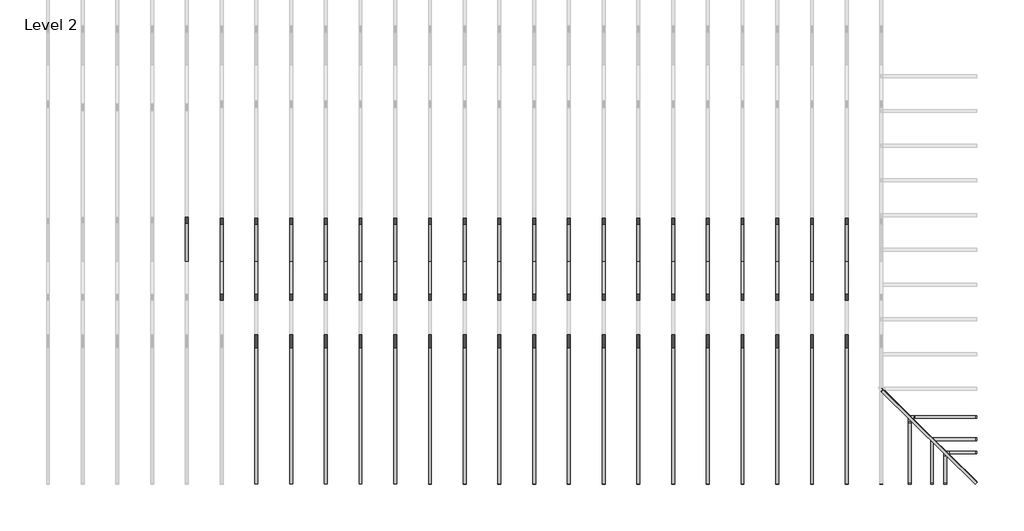
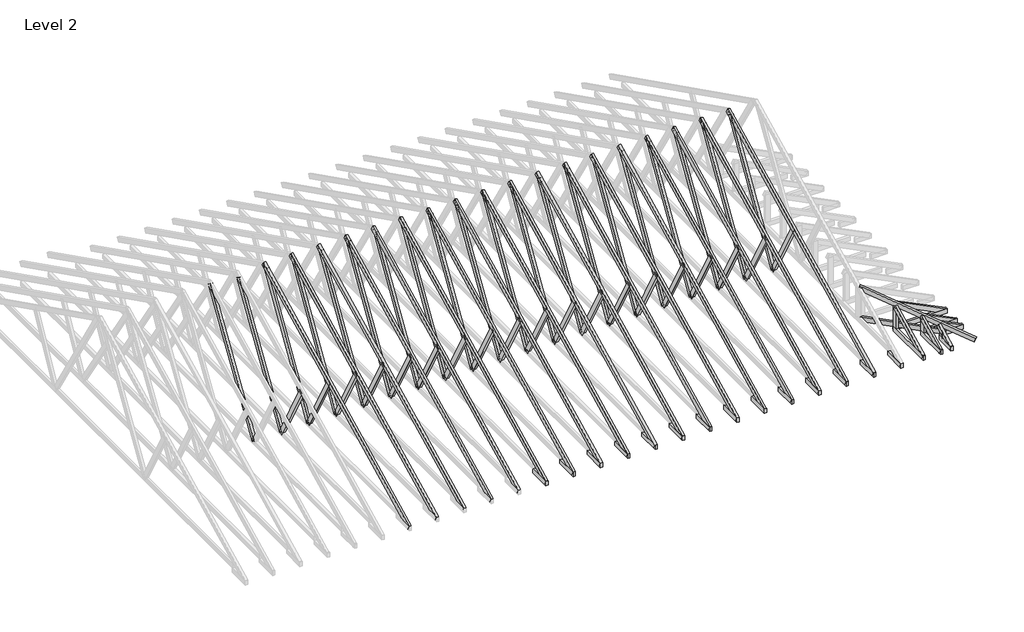
# One storey, part 2 of 5: 91 beams.
"""IFC4 building model written with IfcOpenShell, lengths in millimetres."""

import ifcopenshell
import ifcopenshell.guid

model = None  # the IFC model being written
_history = None  # IfcOwnerHistory: only IFC2X3 demands one
_inside = {}  # id of a spatial element -> (the spatial element, [elements in it])
_under = {}  # id of a project, library or spatial element -> (it, [spatial elements below it])
_declared = {}  # id of a project -> (the project, [libraries it declares])
_typed = {}  # id of a type object -> (the type object, [elements of that type])
_made_of = {}  # id of a material, layer set ... -> (it, [elements and type objects made of it])


def new_model(schema):
    """Start an empty IFC model of exactly this schema.

    Asked for "IFC4X3", IfcOpenShell would pick the latest addendum, in which some entities
    have other attributes; the version numbers below select the first issue.
    IFC2X3 requires an IfcOwnerHistory on every rooted entity: one is made here for all.
    """
    global model, _history
    if schema == "IFC4X3":
        model = ifcopenshell.file(schema_version=(4, 3, 0, 0))
    else:
        model = ifcopenshell.file(schema=schema)
    _inside.clear()
    _under.clear()
    _declared.clear()
    _typed.clear()
    _made_of.clear()
    _history = None
    if model.schema == "IFC2X3":
        org = make("IfcOrganization", Name="unknown")
        user = make(
            "IfcPersonAndOrganization",
            ThePerson=make("IfcPerson", FamilyName="unknown"),
            TheOrganization=org,
        )
        app = make(
            "IfcApplication",
            ApplicationDeveloper=org,
            Version="unknown",
            ApplicationFullName="unknown",
            ApplicationIdentifier="unknown",
        )
        _history = make(
            "IfcOwnerHistory",
            OwningUser=user,
            OwningApplication=app,
            ChangeAction="ADDED",
            CreationDate=0,
        )
    return model


def make(cls, **values):
    """One entity of the class cls with the attributes given. An attribute that is None is left unset."""
    return model.create_entity(
        cls, **{name: value for name, value in values.items() if value is not None}
    )


def rooted(cls, **values):
    """An entity with a GlobalId (a new one), such as an element, a storey or a relation."""
    return make(cls, GlobalId=ifcopenshell.guid.new(), OwnerHistory=_history, **values)


def si_unit(unit_type, name, prefix=None):
    """IfcSIUnit, for example si_unit("LENGTHUNIT", "METRE", prefix="MILLI")."""
    return make("IfcSIUnit", UnitType=unit_type, Prefix=prefix, Name=name)


def assignment(units):
    """IfcUnitAssignment: the units of a project."""
    return None if units is None else make("IfcUnitAssignment", Units=units)


def point(xyz):
    """IfcCartesianPoint."""
    return None if xyz is None else make("IfcCartesianPoint", Coordinates=xyz)


def direction(xyz):
    """IfcDirection."""
    return None if xyz is None else make("IfcDirection", DirectionRatios=xyz)


def frame(location, z_axis=None, x_axis=None):
    """IfcAxis2Placement3D, a coordinate frame: its origin and axes. An axis left out is left unset."""
    return make(
        "IfcAxis2Placement3D",
        Location=point(location),
        Axis=direction(z_axis),
        RefDirection=direction(x_axis),
    )


def origin():
    """The frame at (0, 0, 0) with its axes left unset."""
    return frame((0.0, 0.0, 0.0))


def place(relative_to, where):
    """IfcLocalPlacement: puts the frame where relative to a parent placement (None: the world)."""
    return make(
        "IfcLocalPlacement", PlacementRelTo=relative_to, RelativePlacement=where
    )


def context(
    kind, dimensions, precision=None, world=None, true_north=None, identifier=None
):
    """IfcGeometricRepresentationContext, for example the 3D "Model" context."""
    return make(
        "IfcGeometricRepresentationContext",
        ContextIdentifier=identifier,
        ContextType=kind,
        CoordinateSpaceDimension=dimensions,
        Precision=precision,
        WorldCoordinateSystem=world,
        TrueNorth=true_north,
    )


def project(units=None, contexts=None):
    """IfcProject with its units and contexts."""
    return rooted(
        "IfcProject",
        Name="project",
        RepresentationContexts=contexts,
        UnitsInContext=assignment(units),
    )


def spatial(cls, under=None, at=None, **own):
    """A site, building, storey or space (cls), placed at a placement, below another one or the project."""
    s = rooted(cls, ObjectPlacement=at, **own)
    if under is not None:
        _under.setdefault(under.id(), (under, []))[1].append(s)
    return s


def polyline(points):
    """IfcPolyline through the points."""
    return make("IfcPolyline", Points=[point(p) for p in points])


def outline(outer, holes=None, kind="AREA"):
    """IfcArbitraryClosedProfileDef: a profile drawn as a closed curve; with holes, ...WithVoids."""
    if holes is None:
        return make("IfcArbitraryClosedProfileDef", ProfileType=kind, OuterCurve=outer)
    return make(
        "IfcArbitraryProfileDefWithVoids",
        ProfileType=kind,
        OuterCurve=outer,
        InnerCurves=holes,
    )


def extrude(swept, where, along, depth):
    """IfcExtrudedAreaSolid: the profile swept, set in the frame where, extruded along a direction by depth."""
    return make(
        "IfcExtrudedAreaSolid",
        SweptArea=swept,
        Position=where,
        ExtrudedDirection=direction(along),
        Depth=depth,
    )


def shape(context_of_items, identifier, shape_type, items):
    """IfcShapeRepresentation: the items that make up one representation, for example the "Body"."""
    return make(
        "IfcShapeRepresentation",
        ContextOfItems=context_of_items,
        RepresentationIdentifier=identifier,
        RepresentationType=shape_type,
        Items=items,
    )


def source(mapping_origin, context_of_items, identifier, shape_type, items):
    """IfcRepresentationMap: a shape defined once, which mapped items show again and again."""
    return make(
        "IfcRepresentationMap",
        MappingOrigin=mapping_origin,
        MappedRepresentation=shape(context_of_items, identifier, shape_type, items),
    )


def transform(
    local_origin,
    x_axis=None,
    y_axis=None,
    z_axis=None,
    scale=None,
    scale2=None,
    scale3=None,
    uniform=True,
):
    """IfcCartesianTransformationOperator3D, or its non-uniform kind. x_axis, y_axis, z_axis: its Axis1, 2, 3."""
    if uniform:
        return make(
            "IfcCartesianTransformationOperator3D",
            Axis1=direction(x_axis),
            Axis2=direction(y_axis),
            LocalOrigin=point(local_origin),
            Scale=scale,
            Axis3=direction(z_axis),
        )
    return make(
        "IfcCartesianTransformationOperator3DnonUniform",
        Axis1=direction(x_axis),
        Axis2=direction(y_axis),
        LocalOrigin=point(local_origin),
        Scale=scale,
        Axis3=direction(z_axis),
        Scale2=scale2,
        Scale3=scale3,
    )


def mapped(mapping_source, mapping_target):
    """IfcMappedItem: shows the shape of a source again, moved by a transform."""
    return make(
        "IfcMappedItem", MappingSource=mapping_source, MappingTarget=mapping_target
    )


def made_of(thing, what):
    """Note that an element or type object is made of a material, layer set ...; save() writes the relation."""
    if what is not None:
        _made_of.setdefault(what.id(), (what, []))[1].append(thing)
    return thing


def element(
    cls,
    number,
    at=None,
    inside=None,
    cuts=None,
    type_object=None,
    material=None,
    context=None,
    identifier="Body",
    shape_type=None,
    held_by="IfcProductDefinitionShape",
    body=None,
    shapes=None,
    **own,
):
    """One element of the class cls, such as IfcWall. Its Tag is "e" and its number.

    at: its placement. inside: the storey or other place that contains it. cuts: it is an
    opening in that element (IfcRelVoidsElement). A single representation is given by context,
    identifier, shape_type and body (its items); several are given by shapes. held_by: the class
    of the entity that holds the representations. save() writes the other relations.
    """
    e = rooted(cls, Tag="e%d" % number, ObjectPlacement=at, **own)
    if body is not None:
        shapes = [shape(context, identifier, shape_type, body)]
    if shapes is not None:
        e.Representation = make(held_by, Representations=shapes)
    if inside is not None:
        _inside.setdefault(inside.id(), (inside, []))[1].append(e)
    if cuts is not None:
        rooted(
            "IfcRelVoidsElement", RelatingBuildingElement=cuts, RelatedOpeningElement=e
        )
    if type_object is not None:
        _typed.setdefault(type_object.id(), (type_object, []))[1].append(e)
    return made_of(e, material)


def aggregate(whole, parts):
    """IfcRelAggregates: a whole, such as a stair, and the parts it consists of."""
    return rooted("IfcRelAggregates", RelatingObject=whole, RelatedObjects=parts)


def save(model, path):
    """Write the relations noted so far, then the file.

    IfcRelAggregates (storeys below a building ...), IfcRelContainedInSpatialStructure (elements
    in a storey), IfcRelDefinesByType, IfcRelAssociatesMaterial and IfcRelDeclares: one each for
    every whole, place, type object, material and project.
    """
    for whole, parts in _under.values():
        aggregate(whole, parts)
    for where, things in _inside.values():
        rooted(
            "IfcRelContainedInSpatialStructure",
            RelatedElements=things,
            RelatingStructure=where,
        )
    for kind, things in _typed.values():
        rooted("IfcRelDefinesByType", RelatedObjects=things, RelatingType=kind)
    for what, things in _made_of.values():
        rooted("IfcRelAssociatesMaterial", RelatedObjects=things, RelatingMaterial=what)
    for by, libraries in _declared.values():
        rooted("IfcRelDeclares", RelatingContext=by, RelatedDefinitions=libraries)
    model.write(path)


def beam_3a1eac92(model_context):
    return source(origin(), model_context, "Body", "SweptSolid", [
        extrude(outline(polyline([(233.4866591, 25.4), (233.4866591, -25.4), (-1464.867127, -25.4), (-1464.867127, 25.4), (233.4866591, 25.4)])), frame((0.0, 0.0, -50.8), z_axis=(0.0, 0.0, 1.0), x_axis=(1.0, 0.0, 0.0)), (0.0, 0.0, 1.0), 101.6),
    ])


def beam_7745fe0f(model_context):
    return source(origin(), model_context, "Body", "SweptSolid", [
        extrude(outline(polyline([(393.7, 25.4), (393.7, -25.4), (-393.7, -25.4), (-393.7, 25.4), (393.7, 25.4)])), frame((0.0, 0.0, -50.8), z_axis=(0.0, 0.0, 1.0), x_axis=(1.0, 0.0, 0.0)), (0.0, 0.0, 1.0), 101.6),
    ])


def beam_54dd7b45(model_context):
    return source(origin(), model_context, "Body", "SweptSolid", [
        extrude(outline(polyline([(393.7, -25.4), (-368.3, -25.4), (-368.3, 25.4), (393.7, 25.4), (393.7, -25.4)])), frame((0.0, 0.0, -50.8), z_axis=(0.0, 0.0, 1.0), x_axis=(1.0, 0.0, 0.0)), (0.0, 0.0, 1.0), 101.6),
    ])


def beam_16181373(model_context):
    return source(origin(), model_context, "Body", "SweptSolid", [
        extrude(outline(polyline([(819.5010489, 25.4), (819.5010489, -25.4), (-821.193698, -25.4), (-821.193698, 25.4), (819.5010489, 25.4)])), frame((0.0, 0.0, -50.8), z_axis=(0.0, 0.0, 1.0), x_axis=(1.0, 0.0, 0.0)), (0.0, 0.0, 1.0), 101.6),
    ])


def beam_e838d316(model_context):
    return source(origin(), model_context, "Body", "SweptSolid", [
        extrude(outline(polyline([(1561.1045551, 25.4), (1561.1045551, -25.4), (-1572.5300502, -25.4), (-1572.5300502, 25.4), (1561.1045551, 25.4)])), frame((0.0, 0.0, -50.8), z_axis=(0.0, 0.0, 1.0), x_axis=(1.0, 0.0, 0.0)), (0.0, 0.0, 1.0), 101.6),
    ])


def beam_6a2c9f8f(model_context):
    return source(origin(), model_context, "Body", "SweptSolid", [
        extrude(outline(polyline([(1599.9543138, 25.4), (1599.9543138, -25.4), (-1584.2465686, -25.4), (-1584.2465686, 25.4), (1599.9543138, 25.4)])), frame((0.0, 0.0, -50.8), z_axis=(0.0, 0.0, 1.0), x_axis=(1.0, 0.0, 0.0)), (0.0, 0.0, 1.0), 101.6),
    ])


def beam_87710fdd(model_context):
    return source(origin(), model_context, "Body", "SweptSolid", [
        extrude(outline(polyline([(147.1272806, 25.4), (147.1272806, -25.4), (-142.875, -25.4), (-142.875, 25.4), (147.1272806, 25.4)])), frame((0.0, 0.0, -50.8), z_axis=(0.0, 0.0, 1.0), x_axis=(1.0, 0.0, 0.0)), (0.0, 0.0, 1.0), 101.6),
    ])


def beam_af5d22dc(model_context):
    return source(origin(), model_context, "Body", "SweptSolid", [
        extrude(outline(polyline([(571.5, 25.4), (571.5, -25.4), (-609.6, -25.4), (-609.6, 25.4), (571.5, 25.4)])), frame((0.0, 0.0, -50.8), z_axis=(0.0, 0.0, 1.0), x_axis=(1.0, 0.0, 0.0)), (0.0, 0.0, 1.0), 101.6),
    ])


def beam_7b8fa6d1(model_context):
    return source(origin(), model_context, "Body", "SweptSolid", [
        extrude(outline(polyline([(270.7395597, 25.4), (270.7395597, -25.4), (-219.9395597, -25.4), (-219.9395597, 25.4), (270.7395597, 25.4)])), frame((0.0, 0.0, -50.8), z_axis=(0.0, 0.0, 1.0), x_axis=(1.0, 0.0, 0.0)), (0.0, 0.0, 1.0), 101.6),
    ])


def beam_42a29ae5(model_context):
    return source(origin(), model_context, "Body", "SweptSolid", [
        extrude(outline(polyline([(270.7395597, -25.4), (-219.9395597, -25.4), (-219.9395597, 25.4), (270.7395597, 25.4), (270.7395597, -25.4)])), frame((0.0, 0.0, -50.8), z_axis=(0.0, 0.0, 1.0), x_axis=(1.0, 0.0, 0.0)), (0.0, 0.0, 1.0), 101.6),
    ])


def beam_11c5b8ca(model_context):
    return source(origin(), model_context, "Body", "SweptSolid", [
        extrude(outline(polyline([(147.1272806, -25.4), (-142.875, -25.4), (-142.875, 25.4), (147.1272806, 25.4), (147.1272806, -25.4)])), frame((0.0, 0.0, -50.8), z_axis=(0.0, 0.0, 1.0), x_axis=(1.0, 0.0, 0.0)), (0.0, 0.0, 1.0), 101.6),
    ])


def beam_5ac0b85f(model_context):
    return source(origin(), model_context, "Body", "SweptSolid", [
        extrude(outline(polyline([(571.5, -25.4), (-584.2, -25.4), (-584.2, 25.4), (571.5, 25.4), (571.5, -25.4)])), frame((0.0, 0.0, -50.8), z_axis=(0.0, 0.0, 1.0), x_axis=(1.0, 0.0, 0.0)), (0.0, 0.0, 1.0), 101.6),
    ])


def beam_ec111315(model_context):
    return source(origin(), model_context, "Body", "SweptSolid", [
        extrude(outline(polyline([(279.4, -25.4), (-228.6, -25.4), (-228.6, 25.4), (279.4, 25.4), (279.4, -25.4)])), frame((0.0, 0.0, -50.8), z_axis=(0.0, 0.0, 1.0), x_axis=(1.0, 0.0, 0.0)), (0.0, 0.0, 1.0), 101.6),
    ])


def beam_878446a4(model_context):
    return source(origin(), model_context, "Body", "SweptSolid", [
        extrude(outline(polyline([(63.8057136, 25.4), (63.8057136, -25.4), (-59.553433, -25.4), (-59.553433, 25.4), (63.8057136, 25.4)])), frame((0.0, 0.0, -50.8), z_axis=(0.0, 0.0, 1.0), x_axis=(1.0, 0.0, 0.0)), (0.0, 0.0, 1.0), 101.6),
    ])


def beam_bc99fd75(model_context):
    return source(origin(), model_context, "Body", "SweptSolid", [
        extrude(outline(polyline([(222.3387319, 25.4), (222.3387319, -25.4), (-231.775, -25.4), (-231.775, 25.4), (222.3387319, 25.4)])), frame((0.0, 0.0, -50.8), z_axis=(0.0, 0.0, 1.0), x_axis=(1.0, 0.0, 0.0)), (0.0, 0.0, 1.0), 101.6),
    ])


def beam_efe25585(model_context):
    return source(origin(), model_context, "Body", "SweptSolid", [
        extrude(outline(polyline([(222.3387319, -25.4), (-231.775, -25.4), (-231.775, 25.4), (222.3387319, 25.4), (222.3387319, -25.4)])), frame((0.0, 0.0, -50.8), z_axis=(0.0, 0.0, 1.0), x_axis=(1.0, 0.0, 0.0)), (0.0, 0.0, 1.0), 101.6),
    ])


def beam_dfed05dc(model_context):
    return source(origin(), model_context, "Body", "SweptSolid", [
        extrude(outline(polyline([(63.8057136, -25.4), (-59.553433, -25.4), (-59.553433, 25.4), (63.8057136, 25.4), (63.8057136, -25.4)])), frame((0.0, 0.0, -50.8), z_axis=(0.0, 0.0, 1.0), x_axis=(1.0, 0.0, 0.0)), (0.0, 0.0, 1.0), 101.6),
    ])


model = new_model("IFC4")

# Units and contexts
model_context = context("Model", 3, world=origin())
ifc_project = project(units=[si_unit("LENGTHUNIT", "METRE", prefix="MILLI")], contexts=[model_context])

# Site, building, storey
site = spatial("IfcSite", under=ifc_project)
building = spatial("IfcBuilding", under=site)
storey = spatial("IfcBuildingStorey", under=building, Name="Level 2", Elevation=2768.6)

# Beams
placement = place(None, origin())
element("IfcBeam", 1, ObjectType="Dimension Lumber : BLDG 6241 2X4\" TRUSS MEMBER", at=placement, inside=storey, context=model_context, shape_type="SweptSolid", body=[
    extrude(outline(polyline([(0.0, -50.8), (0.0, 0.0), (6302.3539791, 0.0), (6302.3539791, -50.8), (0.0, -50.8)])), frame((-10511.414829, -5565.5155384, 2678.5857718), z_axis=(0.0, -0.447213595499958, 0.894427190999916), x_axis=(0.0, 0.894427190999916, 0.447213595499958)), (0.0, 0.0, 1.0), 101.6),
])
element("IfcBeam", 2, ObjectType="Dimension Lumber : BLDG 6241 2X4\" TRUSS MEMBER", at=placement, inside=storey, context=model_context, shape_type="SweptSolid", body=[
    extrude(outline(polyline([(0.0, -50.8), (0.0, 0.0), (6302.3539791, 0.0), (6302.3539791, -50.8), (0.0, -50.8)])), frame((-9901.814829, -5565.5155384, 2678.5857718), z_axis=(0.0, -0.447213595499958, 0.894427190999916), x_axis=(0.0, 0.894427190999916, 0.447213595499958)), (0.0, 0.0, 1.0), 101.6),
])
element("IfcBeam", 3, ObjectType="Dimension Lumber : BLDG 6241 2X4\" TRUSS MEMBER", at=placement, inside=storey, context=model_context, shape_type="SweptSolid", body=[
    extrude(outline(polyline([(0.0, -50.8), (0.0, 0.0), (6302.3539791, 0.0), (6302.3539791, -50.8), (0.0, -50.8)])), frame((-9292.214829, -5565.5155384, 2678.5857718), z_axis=(0.0, -0.447213595499958, 0.894427190999916), x_axis=(0.0, 0.894427190999916, 0.447213595499958)), (0.0, 0.0, 1.0), 101.6),
])
element("IfcBeam", 4, ObjectType="Dimension Lumber : BLDG 6241 2X4\" TRUSS MEMBER", at=placement, inside=storey, context=model_context, shape_type="SweptSolid", body=[
    extrude(outline(polyline([(0.0, -50.8), (0.0, 0.0), (6302.3539791, 0.0), (6302.3539791, -50.8), (0.0, -50.8)])), frame((-8682.614829, -5565.5155384, 2678.5857718), z_axis=(0.0, -0.447213595499958, 0.894427190999916), x_axis=(0.0, 0.894427190999916, 0.447213595499958)), (0.0, 0.0, 1.0), 101.6),
])
element("IfcBeam", 5, ObjectType="Dimension Lumber : BLDG 6241 2X4\" TRUSS MEMBER", at=placement, inside=storey, context=model_context, shape_type="SweptSolid", body=[
    extrude(outline(polyline([(0.0, -50.8), (0.0, 0.0), (6302.3539791, 0.0), (6302.3539791, -50.8), (0.0, -50.8)])), frame((-8073.014829, -5565.5155384, 2678.5857718), z_axis=(0.0, -0.447213595499958, 0.894427190999916), x_axis=(0.0, 0.894427190999916, 0.447213595499958)), (0.0, 0.0, 1.0), 101.6),
])
element("IfcBeam", 6, ObjectType="Dimension Lumber : BLDG 6241 2X4\" TRUSS MEMBER", at=placement, inside=storey, context=model_context, shape_type="SweptSolid", body=[
    extrude(outline(polyline([(0.0, -50.8), (0.0, 0.0), (6302.3539791, 0.0), (6302.3539791, -50.8), (0.0, -50.8)])), frame((-7463.414829, -5565.5155384, 2678.5857718), z_axis=(0.0, -0.447213595499958, 0.8944271909999159), x_axis=(0.0, 0.8944271909999159, 0.447213595499958)), (0.0, 0.0, 1.0), 101.6),
])
element("IfcBeam", 7, ObjectType="Dimension Lumber : BLDG 6241 2X4\" TRUSS MEMBER", at=placement, inside=storey, context=model_context, shape_type="SweptSolid", body=[
    extrude(outline(polyline([(0.0, -50.8), (0.0, 0.0), (6302.3539791, 0.0), (6302.3539791, -50.8), (0.0, -50.8)])), frame((-6853.814829, -5565.5155384, 2678.5857718), z_axis=(0.0, -0.44721359549995776, 0.894427190999916), x_axis=(0.0, 0.894427190999916, 0.44721359549995776)), (0.0, 0.0, 1.0), 101.6),
])
element("IfcBeam", 8, ObjectType="Dimension Lumber : BLDG 6241 2X4\" TRUSS MEMBER", at=placement, inside=storey, context=model_context, shape_type="SweptSolid", body=[
    extrude(outline(polyline([(0.0, -50.8), (0.0, 0.0), (6302.3539791, 0.0), (6302.3539791, -50.8), (0.0, -50.8)])), frame((-6244.214829, -5565.5155384, 2678.5857718), z_axis=(0.0, -0.447213595499958, 0.894427190999916), x_axis=(0.0, 0.894427190999916, 0.447213595499958)), (0.0, 0.0, 1.0), 101.6),
])
element("IfcBeam", 9, ObjectType="Dimension Lumber : BLDG 6241 2X4\" TRUSS MEMBER", at=placement, inside=storey, context=model_context, shape_type="SweptSolid", body=[
    extrude(outline(polyline([(0.0, -50.8), (0.0, 0.0), (6302.3539791, 0.0), (6302.3539791, -50.8), (0.0, -50.8)])), frame((-5634.614829, -5565.5155384, 2678.5857718), z_axis=(0.0, -0.447213595499958, 0.894427190999916), x_axis=(0.0, 0.894427190999916, 0.447213595499958)), (0.0, 0.0, 1.0), 101.6),
])
element("IfcBeam", 10, ObjectType="Dimension Lumber : BLDG 6241 2X4\" TRUSS MEMBER", at=placement, inside=storey, context=model_context, shape_type="SweptSolid", body=[
    extrude(outline(polyline([(0.0, -50.8), (0.0, 0.0), (6302.3539791, 0.0), (6302.3539791, -50.8), (0.0, -50.8)])), frame((-5025.014829, -5565.5155384, 2678.5857718), z_axis=(0.0, -0.447213595499958, 0.894427190999916), x_axis=(0.0, 0.894427190999916, 0.447213595499958)), (0.0, 0.0, 1.0), 101.6),
])
element("IfcBeam", 11, ObjectType="Dimension Lumber : BLDG 6241 2X4\" TRUSS MEMBER", at=placement, inside=storey, context=model_context, shape_type="SweptSolid", body=[
    extrude(outline(polyline([(0.0, -50.8), (0.0, 0.0), (6302.3539791, 0.0), (6302.3539791, -50.8), (0.0, -50.8)])), frame((-4415.414829, -5565.5155384, 2678.5857718), z_axis=(0.0, -0.447213595499958, 0.894427190999916), x_axis=(0.0, 0.894427190999916, 0.447213595499958)), (0.0, 0.0, 1.0), 101.6),
])
element("IfcBeam", 12, ObjectType="Dimension Lumber : BLDG 6241 2X4\" TRUSS MEMBER", at=placement, inside=storey, context=model_context, shape_type="SweptSolid", body=[
    extrude(outline(polyline([(0.0, -50.8), (0.0, 0.0), (6302.3539791, 0.0), (6302.3539791, -50.8), (0.0, -50.8)])), frame((-3805.814829, -5565.5155384, 2678.5857718), z_axis=(0.0, -0.447213595499958, 0.894427190999916), x_axis=(0.0, 0.894427190999916, 0.447213595499958)), (0.0, 0.0, 1.0), 101.6),
])
element("IfcBeam", 13, ObjectType="Dimension Lumber : BLDG 6241 2X4\" TRUSS MEMBER", at=placement, inside=storey, context=model_context, shape_type="SweptSolid", body=[
    extrude(outline(polyline([(0.0, -50.8), (0.0, 0.0), (6302.3539791, 0.0), (6302.3539791, -50.8), (0.0, -50.8)])), frame((-3196.214829, -5565.5155384, 2678.5857718), z_axis=(0.0, -0.447213595499958, 0.894427190999916), x_axis=(0.0, 0.894427190999916, 0.447213595499958)), (0.0, 0.0, 1.0), 101.6),
])
element("IfcBeam", 14, ObjectType="Dimension Lumber : BLDG 6241 2X4\" TRUSS MEMBER", at=placement, inside=storey, context=model_context, shape_type="SweptSolid", body=[
    extrude(outline(polyline([(0.0, -50.8), (0.0, 0.0), (6302.3539791, 0.0), (6302.3539791, -50.8), (0.0, -50.8)])), frame((-2586.614829, -5565.5155384, 2678.5857718), z_axis=(0.0, -0.447213595499958, 0.894427190999916), x_axis=(0.0, 0.894427190999916, 0.447213595499958)), (0.0, 0.0, 1.0), 101.6),
])
element("IfcBeam", 15, ObjectType="Dimension Lumber : BLDG 6241 2X4\" TRUSS MEMBER", at=placement, inside=storey, context=model_context, shape_type="SweptSolid", body=[
    extrude(outline(polyline([(0.0, -50.8), (0.0, 0.0), (6302.3539791, 0.0), (6302.3539791, -50.8), (0.0, -50.8)])), frame((-1977.014829, -5565.5155384, 2678.5857718), z_axis=(0.0, -0.447213595499958, 0.894427190999916), x_axis=(0.0, 0.894427190999916, 0.447213595499958)), (0.0, 0.0, 1.0), 101.6),
])
element("IfcBeam", 16, ObjectType="Dimension Lumber : BLDG 6241 2X4\" TRUSS MEMBER", at=placement, inside=storey, context=model_context, shape_type="SweptSolid", body=[
    extrude(outline(polyline([(0.0, -50.8), (0.0, 0.0), (6302.3539791, 0.0), (6302.3539791, -50.8), (0.0, -50.8)])), frame((-1367.414829, -5565.5155384, 2678.5857718), z_axis=(0.0, -0.447213595499958, 0.894427190999916), x_axis=(0.0, 0.894427190999916, 0.447213595499958)), (0.0, 0.0, 1.0), 101.6),
])
element("IfcBeam", 17, ObjectType="Dimension Lumber : BLDG 6241 2X4\" TRUSS MEMBER", at=placement, inside=storey, context=model_context, shape_type="SweptSolid", body=[
    extrude(outline(polyline([(0.0, -50.8), (0.0, 0.0), (6302.3539791, 0.0), (6302.3539791, -50.8), (0.0, -50.8)])), frame((-757.814829, -5565.5155384, 2678.5857718), z_axis=(0.0, -0.447213595499958, 0.8944271909999159), x_axis=(0.0, 0.8944271909999159, 0.447213595499958)), (0.0, 0.0, 1.0), 101.6),
])
element("IfcBeam", 18, ObjectType="Dimension Lumber : BLDG 6241 2X4\" TRUSS MEMBER", at=placement, inside=storey, context=model_context, shape_type="SweptSolid", body=[
    extrude(outline(polyline([(0.0, -50.8), (0.0, 0.0), (6302.3539791, 0.0), (6302.3539791, -50.8), (0.0, -50.8)])), frame((-148.214829, -5565.5155384, 2678.5857718), z_axis=(0.0, -0.44721359549995776, 0.894427190999916), x_axis=(0.0, 0.894427190999916, 0.44721359549995776)), (0.0, 0.0, 1.0), 101.6),
])
element("IfcBeam", 19, ObjectType="Dimension Lumber : BLDG 6241 2X4\" TRUSS MEMBER", at=placement, inside=storey, context=model_context, shape_type="SweptSolid", body=[
    extrude(outline(polyline([(0.0, -50.8000001), (0.0, 0.0), (2461.5286969, -1e-07), (2461.5286969, -50.8), (0.0, -50.8000001)])), frame((497.0810747, -3923.9012552, 3516.9362486), z_axis=(0.22183093198504453, -0.25320527715849106, 0.9416358772018718), x_axis=(0.6716162760239294, -0.6604274920267077, -0.3358081380119639)), (0.0, 0.0, 1.0), 101.6),
])
element("IfcBeam", 20, ObjectType="Dimension Lumber : BLDG 6241 2X4\" TRUSS MEMBER", at=placement, inside=storey, context=model_context, shape_type="SweptSolid", body=[
    extrude(outline(polyline([(0.0, -50.8), (0.0, 0.0), (1203.6219076, 0.0), (1203.6219076, -50.8), (0.0, -50.8)])), frame((2112.5153243, -4456.9715886, 2680.3426701), z_axis=(0.44721359549995937, 0.0, 0.8944271909999152), x_axis=(-0.8944271909999152, 0.0, 0.44721359549995937)), (0.0, 0.0, 1.0), 101.6),
])
element("IfcBeam", 21, ObjectType="Dimension Lumber : BLDG 6241 2X4\" TRUSS MEMBER", at=placement, inside=storey, context=model_context, shape_type="SweptSolid", body=[
    extrude(outline(polyline([(0.0, -50.8), (0.0, 0.0), (844.55, 0.0), (844.55, -50.8), (0.0, -50.8)])), frame((2117.2589031, -4850.6715886, 2677.9708807), z_axis=(0.4472135954999599, 0.0, 0.894427190999915), x_axis=(-0.894427190999915, 0.0, 0.4472135954999599)), (0.0, 0.0, 1.0), 101.6),
])
element("IfcBeam", 22, ObjectType="Dimension Lumber : BLDG 6241 2X4\" TRUSS MEMBER", at=placement, inside=storey, context=model_context, shape_type="SweptSolid", body=[
    extrude(outline(polyline([(0.0, 50.8), (1203.6219076, 50.8), (1203.6219076, 0.0), (0.0, 0.0), (0.0, 50.8)])), frame((1007.485171, -5562.001742, 2680.3426701), z_axis=(0.0, -0.44721359549995937, 0.8944271909999152), x_axis=(0.0, 0.8944271909999152, 0.44721359549995937)), (0.0, 0.0, 1.0), 101.6),
])
element("IfcBeam", 23, ObjectType="Dimension Lumber : BLDG 6241 2X4\" TRUSS MEMBER", at=placement, inside=storey, context=model_context, shape_type="SweptSolid", body=[
    extrude(outline(polyline([(0.0, 50.8), (844.55, 50.8), (844.55, 0.0), (0.0, 0.0), (0.0, 50.8)])), frame((1401.185171, -5566.7453207, 2677.9708807), z_axis=(0.0, -0.4472135954999599, 0.894427190999915), x_axis=(0.0, 0.894427190999915, 0.4472135954999599)), (0.0, 0.0, 1.0), 101.6),
])
element("IfcBeam", 24, ObjectType="Dimension Lumber : BLDG 6241 2X4\" TRUSS MEMBER", at=placement, inside=storey, context=model_context, shape_type="SweptSolid", body=[
    extrude(outline(polyline([(0.0, -50.8), (0.0, 0.0), (546.1, 0.0), (546.1, -50.8), (0.0, -50.8)])), frame((2116.9461224, -5079.2715886, 2678.127271), z_axis=(0.4472135954999593, 0.0, 0.8944271909999153), x_axis=(-0.8944271909999153, 0.0, 0.4472135954999593)), (0.0, 0.0, 1.0), 101.6),
])
element("IfcBeam", 25, ObjectType="Dimension Lumber : BLDG 6241 2X4\" TRUSS MEMBER", at=placement, inside=storey, context=model_context, shape_type="SweptSolid", body=[
    extrude(outline(polyline([(0.0, 50.8), (546.1, 50.8), (546.1, 0.0), (0.0, 0.0), (0.0, 50.8)])), frame((1629.785171, -5566.43254, 2678.127271), z_axis=(0.0, -0.4472135954999592, 0.8944271909999153), x_axis=(0.0, 0.8944271909999153, 0.4472135954999592)), (0.0, 0.0, 1.0), 101.6),
])
beam_shape = beam_3a1eac92(model_context)
element("IfcBeam", 26, ObjectType="Dimension Lumber : BLDG 6241 2X4\" TRUSS MEMBER", at=placement, inside=storey, context=model_context, shape_type="MappedRepresentation", body=[
    mapped(beam_shape, transform((677.285171, -4126.7715886, 2819.4), x_axis=(-0.7071067811865508, 0.7071067811865442, 0.0), y_axis=(-0.7071067811865442, -0.7071067811865508, 0.0), z_axis=(0.0, 0.0, 1.0))),
])
beam_2_shape = beam_7745fe0f(model_context)
element("IfcBeam", 27, ObjectType="Dimension Lumber : BLDG 6241 2X4\" TRUSS MEMBER", at=placement, inside=storey, context=model_context, shape_type="MappedRepresentation", body=[
    mapped(beam_2_shape, transform((1769.485171, -4825.2715886, 2728.7708807), x_axis=(1.0, 0.0, 0.0), y_axis=(0.0, 1.0, 0.0), z_axis=(0.0, 0.0, 1.0))),
])
beam_3_shape = beam_54dd7b45(model_context)
element("IfcBeam", 28, ObjectType="Dimension Lumber : BLDG 6241 2X4\" TRUSS MEMBER", at=placement, inside=storey, context=model_context, shape_type="MappedRepresentation", body=[
    mapped(beam_3_shape, transform((1375.785171, -5218.9715886, 2728.7708807), x_axis=(0.0, -1.0, 0.0), y_axis=(1.0, 0.0, 0.0), z_axis=(0.0, 0.0, 1.0))),
])
beam_4_shape = beam_16181373(model_context)
element("IfcBeam", 29, ObjectType="Dimension Lumber : BLDG 6241 2X4\" TRUSS MEMBER", at=placement, inside=storey, context=model_context, shape_type="MappedRepresentation", body=[
    mapped(beam_4_shape, transform((-11095.614829, -2095.6213634, 3552.5770493), x_axis=(0.0, -0.4803172630852174, 0.8770948220017754), y_axis=(-1.0, 0.0, 0.0), z_axis=(0.0, -0.8770948220017754, -0.4803172630852174))),
])
element("IfcBeam", 30, ObjectType="Dimension Lumber : BLDG 6241 2X4\" TRUSS MEMBER", at=placement, inside=storey, context=model_context, shape_type="MappedRepresentation", body=[
    mapped(beam_4_shape, transform((-10486.014829, -2095.6213634, 3552.5770493), x_axis=(0.0, -0.4803172630852174, 0.8770948220017754), y_axis=(-1.0, 0.0, 0.0), z_axis=(0.0, -0.8770948220017754, -0.4803172630852174))),
])
element("IfcBeam", 31, ObjectType="Dimension Lumber : BLDG 6241 2X4\" TRUSS MEMBER", at=placement, inside=storey, context=model_context, shape_type="MappedRepresentation", body=[
    mapped(beam_4_shape, transform((-9876.414829, -2095.6213634, 3552.5770493), x_axis=(0.0, -0.4803172630852174, 0.8770948220017754), y_axis=(-1.0, 0.0, 0.0), z_axis=(0.0, -0.8770948220017754, -0.4803172630852174))),
])
element("IfcBeam", 32, ObjectType="Dimension Lumber : BLDG 6241 2X4\" TRUSS MEMBER", at=placement, inside=storey, context=model_context, shape_type="MappedRepresentation", body=[
    mapped(beam_4_shape, transform((-9266.814829, -2095.6213634, 3552.5770493), x_axis=(0.0, -0.4803172630852174, 0.8770948220017754), y_axis=(-1.0, 0.0, 0.0), z_axis=(0.0, -0.8770948220017754, -0.4803172630852174))),
])
element("IfcBeam", 33, ObjectType="Dimension Lumber : BLDG 6241 2X4\" TRUSS MEMBER", at=placement, inside=storey, context=model_context, shape_type="MappedRepresentation", body=[
    mapped(beam_4_shape, transform((-8657.214829, -2095.6213634, 3552.5770493), x_axis=(0.0, -0.4803172630852174, 0.8770948220017754), y_axis=(-1.0, 0.0, 0.0), z_axis=(0.0, -0.8770948220017754, -0.4803172630852174))),
])
element("IfcBeam", 34, ObjectType="Dimension Lumber : BLDG 6241 2X4\" TRUSS MEMBER", at=placement, inside=storey, context=model_context, shape_type="MappedRepresentation", body=[
    mapped(beam_4_shape, transform((-8047.614829, -2095.6213634, 3552.5770493), x_axis=(0.0, -0.4803172630852174, 0.8770948220017754), y_axis=(-1.0, 0.0, 0.0), z_axis=(0.0, -0.8770948220017754, -0.4803172630852174))),
])
element("IfcBeam", 35, ObjectType="Dimension Lumber : BLDG 6241 2X4\" TRUSS MEMBER", at=placement, inside=storey, context=model_context, shape_type="MappedRepresentation", body=[
    mapped(beam_4_shape, transform((-7438.014829, -2095.6213634, 3552.5770493), x_axis=(0.0, -0.4803172630852174, 0.8770948220017754), y_axis=(-1.0, 0.0, 0.0), z_axis=(0.0, -0.8770948220017754, -0.4803172630852174))),
])
element("IfcBeam", 36, ObjectType="Dimension Lumber : BLDG 6241 2X4\" TRUSS MEMBER", at=placement, inside=storey, context=model_context, shape_type="MappedRepresentation", body=[
    mapped(beam_4_shape, transform((-6828.414829, -2095.6213634, 3552.5770493), x_axis=(0.0, -0.4803172630852174, 0.8770948220017754), y_axis=(-1.0, 0.0, 0.0), z_axis=(0.0, -0.8770948220017754, -0.4803172630852174))),
])
element("IfcBeam", 37, ObjectType="Dimension Lumber : BLDG 6241 2X4\" TRUSS MEMBER", at=placement, inside=storey, context=model_context, shape_type="MappedRepresentation", body=[
    mapped(beam_4_shape, transform((-6218.814829, -2095.6213634, 3552.5770493), x_axis=(0.0, -0.4803172630852174, 0.8770948220017754), y_axis=(-1.0, 0.0, 0.0), z_axis=(0.0, -0.8770948220017754, -0.4803172630852174))),
])
element("IfcBeam", 38, ObjectType="Dimension Lumber : BLDG 6241 2X4\" TRUSS MEMBER", at=placement, inside=storey, context=model_context, shape_type="MappedRepresentation", body=[
    mapped(beam_4_shape, transform((-5609.214829, -2095.6213634, 3552.5770493), x_axis=(0.0, -0.4803172630852174, 0.8770948220017754), y_axis=(-1.0, 0.0, 0.0), z_axis=(0.0, -0.8770948220017754, -0.4803172630852174))),
])
element("IfcBeam", 39, ObjectType="Dimension Lumber : BLDG 6241 2X4\" TRUSS MEMBER", at=placement, inside=storey, context=model_context, shape_type="MappedRepresentation", body=[
    mapped(beam_4_shape, transform((-4999.614829, -2095.6213634, 3552.5770493), x_axis=(0.0, -0.4803172630852174, 0.8770948220017754), y_axis=(-1.0, 0.0, 0.0), z_axis=(0.0, -0.8770948220017754, -0.4803172630852174))),
])
element("IfcBeam", 40, ObjectType="Dimension Lumber : BLDG 6241 2X4\" TRUSS MEMBER", at=placement, inside=storey, context=model_context, shape_type="MappedRepresentation", body=[
    mapped(beam_4_shape, transform((-4390.014829, -2095.6213634, 3552.5770493), x_axis=(0.0, -0.4803172630852174, 0.8770948220017754), y_axis=(-1.0, 0.0, 0.0), z_axis=(0.0, -0.8770948220017754, -0.4803172630852174))),
])
element("IfcBeam", 41, ObjectType="Dimension Lumber : BLDG 6241 2X4\" TRUSS MEMBER", at=placement, inside=storey, context=model_context, shape_type="MappedRepresentation", body=[
    mapped(beam_4_shape, transform((-3780.414829, -2095.6213634, 3552.5770493), x_axis=(0.0, -0.4803172630852174, 0.8770948220017754), y_axis=(-1.0, 0.0, 0.0), z_axis=(0.0, -0.8770948220017754, -0.4803172630852174))),
])
element("IfcBeam", 42, ObjectType="Dimension Lumber : BLDG 6241 2X4\" TRUSS MEMBER", at=placement, inside=storey, context=model_context, shape_type="MappedRepresentation", body=[
    mapped(beam_4_shape, transform((-3170.814829, -2095.6213634, 3552.5770493), x_axis=(0.0, -0.4803172630852174, 0.8770948220017754), y_axis=(-1.0, 0.0, 0.0), z_axis=(0.0, -0.8770948220017754, -0.4803172630852174))),
])
element("IfcBeam", 43, ObjectType="Dimension Lumber : BLDG 6241 2X4\" TRUSS MEMBER", at=placement, inside=storey, context=model_context, shape_type="MappedRepresentation", body=[
    mapped(beam_4_shape, transform((-2561.214829, -2095.6213634, 3552.5770493), x_axis=(0.0, -0.4803172630852174, 0.8770948220017754), y_axis=(-1.0, 0.0, 0.0), z_axis=(0.0, -0.8770948220017754, -0.4803172630852174))),
])
element("IfcBeam", 44, ObjectType="Dimension Lumber : BLDG 6241 2X4\" TRUSS MEMBER", at=placement, inside=storey, context=model_context, shape_type="MappedRepresentation", body=[
    mapped(beam_4_shape, transform((-1951.614829, -2095.6213634, 3552.5770493), x_axis=(0.0, -0.4803172630852174, 0.8770948220017754), y_axis=(-1.0, 0.0, 0.0), z_axis=(0.0, -0.8770948220017754, -0.4803172630852174))),
])
element("IfcBeam", 45, ObjectType="Dimension Lumber : BLDG 6241 2X4\" TRUSS MEMBER", at=placement, inside=storey, context=model_context, shape_type="MappedRepresentation", body=[
    mapped(beam_4_shape, transform((-1342.014829, -2095.6213634, 3552.5770493), x_axis=(0.0, -0.4803172630852174, 0.8770948220017754), y_axis=(-1.0, 0.0, 0.0), z_axis=(0.0, -0.8770948220017754, -0.4803172630852174))),
])
element("IfcBeam", 46, ObjectType="Dimension Lumber : BLDG 6241 2X4\" TRUSS MEMBER", at=placement, inside=storey, context=model_context, shape_type="MappedRepresentation", body=[
    mapped(beam_4_shape, transform((-732.414829, -2095.6213634, 3552.5770493), x_axis=(0.0, -0.4803172630852174, 0.8770948220017754), y_axis=(-1.0, 0.0, 0.0), z_axis=(0.0, -0.8770948220017754, -0.4803172630852174))),
])
element("IfcBeam", 47, ObjectType="Dimension Lumber : BLDG 6241 2X4\" TRUSS MEMBER", at=placement, inside=storey, context=model_context, shape_type="MappedRepresentation", body=[
    mapped(beam_4_shape, transform((-122.814829, -2095.6213634, 3552.5770493), x_axis=(0.0, -0.4803172630852174, 0.8770948220017754), y_axis=(-1.0, 0.0, 0.0), z_axis=(0.0, -0.8770948220017754, -0.4803172630852174))),
])
beam_5_shape = beam_e838d316(model_context)
element("IfcBeam", 48, ObjectType="Dimension Lumber : BLDG 6241 2X4\" TRUSS MEMBER", at=placement, inside=storey, context=model_context, shape_type="MappedRepresentation", body=[
    mapped(beam_5_shape, transform((-11095.614829, -880.0831247, 4160.3461686), x_axis=(0.0, -0.5257715142502325, -0.8506258371358218), y_axis=(-1.0, 0.0, 0.0), z_axis=(0.0, 0.8506258371358218, -0.5257715142502325))),
])
element("IfcBeam", 49, ObjectType="Dimension Lumber : BLDG 6241 2X4\" TRUSS MEMBER", at=placement, inside=storey, context=model_context, shape_type="MappedRepresentation", body=[
    mapped(beam_5_shape, transform((-10486.014829, -880.0831247, 4160.3461686), x_axis=(0.0, -0.5257715142502325, -0.8506258371358218), y_axis=(-1.0, 0.0, 0.0), z_axis=(0.0, 0.8506258371358218, -0.5257715142502325))),
])
element("IfcBeam", 50, ObjectType="Dimension Lumber : BLDG 6241 2X4\" TRUSS MEMBER", at=placement, inside=storey, context=model_context, shape_type="MappedRepresentation", body=[
    mapped(beam_5_shape, transform((-9876.414829, -880.0831247, 4160.3461686), x_axis=(0.0, -0.5257715142502325, -0.8506258371358218), y_axis=(-1.0, 0.0, 0.0), z_axis=(0.0, 0.8506258371358218, -0.5257715142502325))),
])
element("IfcBeam", 51, ObjectType="Dimension Lumber : BLDG 6241 2X4\" TRUSS MEMBER", at=placement, inside=storey, context=model_context, shape_type="MappedRepresentation", body=[
    mapped(beam_5_shape, transform((-9266.814829, -880.0831247, 4160.3461686), x_axis=(0.0, -0.5257715142502325, -0.8506258371358218), y_axis=(-1.0, 0.0, 0.0), z_axis=(0.0, 0.8506258371358218, -0.5257715142502325))),
])
element("IfcBeam", 52, ObjectType="Dimension Lumber : BLDG 6241 2X4\" TRUSS MEMBER", at=placement, inside=storey, context=model_context, shape_type="MappedRepresentation", body=[
    mapped(beam_5_shape, transform((-8657.214829, -880.0831247, 4160.3461686), x_axis=(0.0, -0.5257715142502325, -0.8506258371358218), y_axis=(-1.0, 0.0, 0.0), z_axis=(0.0, 0.8506258371358218, -0.5257715142502325))),
])
element("IfcBeam", 53, ObjectType="Dimension Lumber : BLDG 6241 2X4\" TRUSS MEMBER", at=placement, inside=storey, context=model_context, shape_type="MappedRepresentation", body=[
    mapped(beam_5_shape, transform((-8047.614829, -880.0831247, 4160.3461686), x_axis=(0.0, -0.5257715142502325, -0.8506258371358218), y_axis=(-1.0, 0.0, 0.0), z_axis=(0.0, 0.8506258371358218, -0.5257715142502325))),
])
element("IfcBeam", 54, ObjectType="Dimension Lumber : BLDG 6241 2X4\" TRUSS MEMBER", at=placement, inside=storey, context=model_context, shape_type="MappedRepresentation", body=[
    mapped(beam_5_shape, transform((-7438.014829, -880.0831247, 4160.3461686), x_axis=(0.0, -0.5257715142502325, -0.8506258371358218), y_axis=(-1.0, 0.0, 0.0), z_axis=(0.0, 0.8506258371358218, -0.5257715142502325))),
])
element("IfcBeam", 55, ObjectType="Dimension Lumber : BLDG 6241 2X4\" TRUSS MEMBER", at=placement, inside=storey, context=model_context, shape_type="MappedRepresentation", body=[
    mapped(beam_5_shape, transform((-6828.414829, -880.0831247, 4160.3461686), x_axis=(0.0, -0.5257715142502325, -0.8506258371358218), y_axis=(-1.0, 0.0, 0.0), z_axis=(0.0, 0.8506258371358218, -0.5257715142502325))),
])
element("IfcBeam", 56, ObjectType="Dimension Lumber : BLDG 6241 2X4\" TRUSS MEMBER", at=placement, inside=storey, context=model_context, shape_type="MappedRepresentation", body=[
    mapped(beam_5_shape, transform((-6218.814829, -880.0831247, 4160.3461686), x_axis=(0.0, -0.5257715142502325, -0.8506258371358218), y_axis=(-1.0, 0.0, 0.0), z_axis=(0.0, 0.8506258371358218, -0.5257715142502325))),
])
element("IfcBeam", 57, ObjectType="Dimension Lumber : BLDG 6241 2X4\" TRUSS MEMBER", at=placement, inside=storey, context=model_context, shape_type="MappedRepresentation", body=[
    mapped(beam_5_shape, transform((-5609.214829, -880.0831247, 4160.3461686), x_axis=(0.0, -0.5257715142502325, -0.8506258371358218), y_axis=(-1.0, 0.0, 0.0), z_axis=(0.0, 0.8506258371358218, -0.5257715142502325))),
])
element("IfcBeam", 58, ObjectType="Dimension Lumber : BLDG 6241 2X4\" TRUSS MEMBER", at=placement, inside=storey, context=model_context, shape_type="MappedRepresentation", body=[
    mapped(beam_5_shape, transform((-4999.614829, -880.0831247, 4160.3461686), x_axis=(0.0, -0.5257715142502325, -0.8506258371358218), y_axis=(-1.0, 0.0, 0.0), z_axis=(0.0, 0.8506258371358218, -0.5257715142502325))),
])
element("IfcBeam", 59, ObjectType="Dimension Lumber : BLDG 6241 2X4\" TRUSS MEMBER", at=placement, inside=storey, context=model_context, shape_type="MappedRepresentation", body=[
    mapped(beam_5_shape, transform((-4390.014829, -880.0831247, 4160.3461686), x_axis=(0.0, -0.5257715142502325, -0.8506258371358218), y_axis=(-1.0, 0.0, 0.0), z_axis=(0.0, 0.8506258371358218, -0.5257715142502325))),
])
element("IfcBeam", 60, ObjectType="Dimension Lumber : BLDG 6241 2X4\" TRUSS MEMBER", at=placement, inside=storey, context=model_context, shape_type="MappedRepresentation", body=[
    mapped(beam_5_shape, transform((-3780.414829, -880.0831247, 4160.3461686), x_axis=(0.0, -0.5257715142502325, -0.8506258371358218), y_axis=(-1.0, 0.0, 0.0), z_axis=(0.0, 0.8506258371358218, -0.5257715142502325))),
])
element("IfcBeam", 61, ObjectType="Dimension Lumber : BLDG 6241 2X4\" TRUSS MEMBER", at=placement, inside=storey, context=model_context, shape_type="MappedRepresentation", body=[
    mapped(beam_5_shape, transform((-3170.814829, -880.0831247, 4160.3461686), x_axis=(0.0, -0.5257715142502325, -0.8506258371358218), y_axis=(-1.0, 0.0, 0.0), z_axis=(0.0, 0.8506258371358218, -0.5257715142502325))),
])
element("IfcBeam", 62, ObjectType="Dimension Lumber : BLDG 6241 2X4\" TRUSS MEMBER", at=placement, inside=storey, context=model_context, shape_type="MappedRepresentation", body=[
    mapped(beam_5_shape, transform((-2561.214829, -880.0831247, 4160.3461686), x_axis=(0.0, -0.5257715142502325, -0.8506258371358218), y_axis=(-1.0, 0.0, 0.0), z_axis=(0.0, 0.8506258371358218, -0.5257715142502325))),
])
element("IfcBeam", 63, ObjectType="Dimension Lumber : BLDG 6241 2X4\" TRUSS MEMBER", at=placement, inside=storey, context=model_context, shape_type="MappedRepresentation", body=[
    mapped(beam_5_shape, transform((-1951.614829, -880.0831247, 4160.3461686), x_axis=(0.0, -0.5257715142502325, -0.8506258371358218), y_axis=(-1.0, 0.0, 0.0), z_axis=(0.0, 0.8506258371358218, -0.5257715142502325))),
])
element("IfcBeam", 64, ObjectType="Dimension Lumber : BLDG 6241 2X4\" TRUSS MEMBER", at=placement, inside=storey, context=model_context, shape_type="MappedRepresentation", body=[
    mapped(beam_5_shape, transform((-1342.014829, -880.0831247, 4160.3461686), x_axis=(0.0, -0.5257715142502325, -0.8506258371358218), y_axis=(-1.0, 0.0, 0.0), z_axis=(0.0, 0.8506258371358218, -0.5257715142502325))),
])
element("IfcBeam", 65, ObjectType="Dimension Lumber : BLDG 6241 2X4\" TRUSS MEMBER", at=placement, inside=storey, context=model_context, shape_type="MappedRepresentation", body=[
    mapped(beam_5_shape, transform((-732.414829, -880.0831247, 4160.3461686), x_axis=(0.0, -0.5257715142502325, -0.8506258371358218), y_axis=(-1.0, 0.0, 0.0), z_axis=(0.0, 0.8506258371358218, -0.5257715142502325))),
])
element("IfcBeam", 66, ObjectType="Dimension Lumber : BLDG 6241 2X4\" TRUSS MEMBER", at=placement, inside=storey, context=model_context, shape_type="MappedRepresentation", body=[
    mapped(beam_5_shape, transform((-122.814829, -880.0831247, 4160.3461686), x_axis=(0.0, -0.5257715142502325, -0.8506258371358218), y_axis=(-1.0, 0.0, 0.0), z_axis=(0.0, 0.8506258371358218, -0.5257715142502325))),
])
beam_6_shape = beam_6a2c9f8f(model_context)
element("IfcBeam", 67, ObjectType="Dimension Lumber : BLDG 6241 2X4\" TRUSS MEMBER", at=placement, inside=storey, context=model_context, shape_type="MappedRepresentation", body=[
    mapped(beam_6_shape, transform((-11705.214829, -844.5384628, 4185.1853738), x_axis=(0.0, -0.5348644598757986, -0.8449378731964677), y_axis=(-1.0, 0.0, 0.0), z_axis=(0.0, 0.8449378731964677, -0.5348644598757986))),
])
beam_7_shape = beam_87710fdd(model_context)
element("IfcBeam", 68, ObjectType="Dimension Lumber : BLDG 6241 2X4\" TRUSS MEMBER", at=placement, inside=storey, context=model_context, shape_type="MappedRepresentation", body=[
    mapped(beam_7_shape, transform((1451.985171, -4825.2715886, 2924.5288734), x_axis=(0.0, 0.0, 1.0), y_axis=(0.0, -1.0, 0.0), z_axis=(1.0, 0.0, 0.0))),
])
beam_8_shape = beam_af5d22dc(model_context)
element("IfcBeam", 69, ObjectType="Dimension Lumber : BLDG 6241 2X4\" TRUSS MEMBER", at=placement, inside=storey, context=model_context, shape_type="MappedRepresentation", body=[
    mapped(beam_8_shape, transform((1591.685171, -4431.5715886, 2728.7708807), x_axis=(1.0, 0.0, 0.0), y_axis=(0.0, 1.0, 0.0), z_axis=(0.0, 0.0, 1.0))),
])
beam_9_shape = beam_7b8fa6d1(model_context)
element("IfcBeam", 70, ObjectType="Dimension Lumber : BLDG 6241 2X4\" TRUSS MEMBER", at=placement, inside=storey, context=model_context, shape_type="MappedRepresentation", body=[
    mapped(beam_9_shape, transform((1058.285171, -4431.5715886, 2999.5104403), x_axis=(0.0, 0.0, 1.0), y_axis=(0.0, -1.0, 0.0), z_axis=(1.0, 0.0, 0.0))),
])
beam_10_shape = beam_42a29ae5(model_context)
element("IfcBeam", 71, ObjectType="Dimension Lumber : BLDG 6241 2X4\" TRUSS MEMBER", at=placement, inside=storey, context=model_context, shape_type="MappedRepresentation", body=[
    mapped(beam_10_shape, transform((982.085171, -4507.7715886, 2999.5104403), x_axis=(0.0, 0.0, 1.0), y_axis=(-1.0, 0.0, 0.0), z_axis=(0.0, -1.0, 0.0))),
])
beam_11_shape = beam_11c5b8ca(model_context)
element("IfcBeam", 72, ObjectType="Dimension Lumber : BLDG 6241 2X4\" TRUSS MEMBER", at=placement, inside=storey, context=model_context, shape_type="MappedRepresentation", body=[
    mapped(beam_11_shape, transform((1375.785171, -4901.4715886, 2924.5288734), x_axis=(0.0, 0.0, 1.0), y_axis=(-1.0, 0.0, 0.0), z_axis=(0.0, -1.0, 0.0))),
])
beam_12_shape = beam_5ac0b85f(model_context)
element("IfcBeam", 73, ObjectType="Dimension Lumber : BLDG 6241 2X4\" TRUSS MEMBER", at=placement, inside=storey, context=model_context, shape_type="MappedRepresentation", body=[
    mapped(beam_12_shape, transform((982.085171, -5041.1715886, 2728.7708807), x_axis=(0.0, -1.0, 0.0), y_axis=(1.0, 0.0, 0.0), z_axis=(0.0, 0.0, 1.0))),
])
beam_13_shape = beam_ec111315(model_context)
element("IfcBeam", 74, ObjectType="Dimension Lumber : BLDG 6241 2X4\" TRUSS MEMBER", at=placement, inside=storey, context=model_context, shape_type="MappedRepresentation", body=[
    mapped(beam_13_shape, transform((-7438.014829, -5384.0715886, 2717.8), x_axis=(0.0, 1.0, 0.0), y_axis=(-1.0, 0.0, 0.0), z_axis=(0.0, 0.0, 1.0))),
])
element("IfcBeam", 75, ObjectType="Dimension Lumber : BLDG 6241 2X4\" TRUSS MEMBER", at=placement, inside=storey, context=model_context, shape_type="MappedRepresentation", body=[
    mapped(beam_13_shape, transform((-6828.414829, -5384.0715886, 2717.8), x_axis=(0.0, 1.0, 0.0), y_axis=(-1.0, 0.0, 0.0), z_axis=(0.0, 0.0, 1.0))),
])
element("IfcBeam", 76, ObjectType="Dimension Lumber : BLDG 6241 2X4\" TRUSS MEMBER", at=placement, inside=storey, context=model_context, shape_type="MappedRepresentation", body=[
    mapped(beam_13_shape, transform((-6218.814829, -5384.0715886, 2717.8), x_axis=(0.0, 1.0, 0.0), y_axis=(-1.0, 0.0, 0.0), z_axis=(0.0, 0.0, 1.0))),
])
element("IfcBeam", 77, ObjectType="Dimension Lumber : BLDG 6241 2X4\" TRUSS MEMBER", at=placement, inside=storey, context=model_context, shape_type="MappedRepresentation", body=[
    mapped(beam_13_shape, transform((-5609.214829, -5384.0715886, 2717.8), x_axis=(0.0, 1.0, 0.0), y_axis=(-1.0, 0.0, 0.0), z_axis=(0.0, 0.0, 1.0))),
])
element("IfcBeam", 78, ObjectType="Dimension Lumber : BLDG 6241 2X4\" TRUSS MEMBER", at=placement, inside=storey, context=model_context, shape_type="MappedRepresentation", body=[
    mapped(beam_13_shape, transform((-4999.614829, -5384.0715886, 2717.8), x_axis=(0.0, 1.0, 0.0), y_axis=(-1.0, 0.0, 0.0), z_axis=(0.0, 0.0, 1.0))),
])
element("IfcBeam", 79, ObjectType="Dimension Lumber : BLDG 6241 2X4\" TRUSS MEMBER", at=placement, inside=storey, context=model_context, shape_type="MappedRepresentation", body=[
    mapped(beam_13_shape, transform((-4390.014829, -5384.0715886, 2717.8), x_axis=(0.0, 1.0, 0.0), y_axis=(-1.0, 0.0, 0.0), z_axis=(0.0, 0.0, 1.0))),
])
element("IfcBeam", 80, ObjectType="Dimension Lumber : BLDG 6241 2X4\" TRUSS MEMBER", at=placement, inside=storey, context=model_context, shape_type="MappedRepresentation", body=[
    mapped(beam_13_shape, transform((-3780.414829, -5384.0715886, 2717.8), x_axis=(0.0, 1.0, 0.0), y_axis=(-1.0, 0.0, 0.0), z_axis=(0.0, 0.0, 1.0))),
])
element("IfcBeam", 81, ObjectType="Dimension Lumber : BLDG 6241 2X4\" TRUSS MEMBER", at=placement, inside=storey, context=model_context, shape_type="MappedRepresentation", body=[
    mapped(beam_13_shape, transform((-3170.814829, -5384.0715886, 2717.8), x_axis=(0.0, 1.0, 0.0), y_axis=(-1.0, 0.0, 0.0), z_axis=(0.0, 0.0, 1.0))),
])
element("IfcBeam", 82, ObjectType="Dimension Lumber : BLDG 6241 2X4\" TRUSS MEMBER", at=placement, inside=storey, context=model_context, shape_type="MappedRepresentation", body=[
    mapped(beam_13_shape, transform((-2561.214829, -5384.0715886, 2717.8), x_axis=(0.0, 1.0, 0.0), y_axis=(-1.0, 0.0, 0.0), z_axis=(0.0, 0.0, 1.0))),
])
element("IfcBeam", 83, ObjectType="Dimension Lumber : BLDG 6241 2X4\" TRUSS MEMBER", at=placement, inside=storey, context=model_context, shape_type="MappedRepresentation", body=[
    mapped(beam_13_shape, transform((-1951.614829, -5384.0715886, 2717.8), x_axis=(0.0, 1.0, 0.0), y_axis=(-1.0, 0.0, 0.0), z_axis=(0.0, 0.0, 1.0))),
])
element("IfcBeam", 84, ObjectType="Dimension Lumber : BLDG 6241 2X4\" TRUSS MEMBER", at=placement, inside=storey, context=model_context, shape_type="MappedRepresentation", body=[
    mapped(beam_13_shape, transform((-1342.014829, -5384.0715886, 2717.8), x_axis=(0.0, 1.0, 0.0), y_axis=(-1.0, 0.0, 0.0), z_axis=(0.0, 0.0, 1.0))),
])
element("IfcBeam", 85, ObjectType="Dimension Lumber : BLDG 6241 2X4\" TRUSS MEMBER", at=placement, inside=storey, context=model_context, shape_type="MappedRepresentation", body=[
    mapped(beam_13_shape, transform((-732.414829, -5384.0715886, 2717.8), x_axis=(0.0, 1.0, 0.0), y_axis=(-1.0, 0.0, 0.0), z_axis=(0.0, 0.0, 1.0))),
])
element("IfcBeam", 86, ObjectType="Dimension Lumber : BLDG 6241 2X4\" TRUSS MEMBER", at=placement, inside=storey, context=model_context, shape_type="MappedRepresentation", body=[
    mapped(beam_13_shape, transform((-122.814829, -5384.0715886, 2717.8), x_axis=(0.0, 1.0, 0.0), y_axis=(-1.0, 0.0, 0.0), z_axis=(0.0, 0.0, 1.0))),
])
element("IfcBeam", 87, ObjectType="Dimension Lumber : BLDG 6241 2X4\" TRUSS MEMBER", at=placement, inside=storey, context=model_context, shape_type="MappedRepresentation", body=[
    mapped(beam_13_shape, transform((486.785171, -5384.0715886, 2717.8), x_axis=(0.0, 1.0, 0.0), y_axis=(-1.0, 0.0, 0.0), z_axis=(0.0, 0.0, 1.0))),
])
beam_14_shape = beam_878446a4(model_context)
element("IfcBeam", 88, ObjectType="Dimension Lumber : BLDG 6241 2X4\" TRUSS MEMBER", at=placement, inside=storey, context=model_context, shape_type="MappedRepresentation", body=[
    mapped(beam_14_shape, transform((1785.271439, -5053.8715886, 2841.2073064), x_axis=(0.0, 0.0, 1.0), y_axis=(0.0, -1.0, 0.0), z_axis=(1.0, 0.0, 0.0))),
])
beam_15_shape = beam_bc99fd75(model_context)
element("IfcBeam", 89, ObjectType="Dimension Lumber : BLDG 6241 2X4\" TRUSS MEMBER", at=placement, inside=storey, context=model_context, shape_type="MappedRepresentation", body=[
    mapped(beam_15_shape, transform((1940.846439, -5053.8715886, 2728.7708807), x_axis=(1.0, 0.0, 0.0), y_axis=(0.0, 1.0, 0.0), z_axis=(0.0, 0.0, 1.0))),
])
beam_16_shape = beam_efe25585(model_context)
element("IfcBeam", 90, ObjectType="Dimension Lumber : BLDG 6241 2X4\" TRUSS MEMBER", at=placement, inside=storey, context=model_context, shape_type="MappedRepresentation", body=[
    mapped(beam_16_shape, transform((1604.385171, -5390.3328567, 2728.7708807), x_axis=(0.0, -1.0, 0.0), y_axis=(1.0, 0.0, 0.0), z_axis=(0.0, 0.0, 1.0))),
])
beam_17_shape = beam_dfed05dc(model_context)
element("IfcBeam", 91, ObjectType="Dimension Lumber : BLDG 6241 2X4\" TRUSS MEMBER", at=placement, inside=storey, context=model_context, shape_type="MappedRepresentation", body=[
    mapped(beam_17_shape, transform((1604.385171, -5234.7578567, 2841.2073064), x_axis=(0.0, 0.0, 1.0), y_axis=(-1.0, 0.0, 0.0), z_axis=(0.0, -1.0, 0.0))),
])

save(model, "model.ifc")

# Revit data of these elements
# Type "Dimension Lumber : BLDG 6241 2X4\" TRUSS MEMBER"
#   Assembly Code = "B10"
#   A = 0.273472 SF
#   Length [instance default] = 5' - 0"
#   b = 0' - 2"
#   d = 0' - 4"
#   Structural Material [instance default] = Softwood, Lumber
# Elements 1, 2, 3, 4, 5, 6, 7, 8, 9, 10, 11, 12, 13, 14, 15, 16, 17, 18, 19, 20, 21, 22, 23, 24, 25, 26, 27, 28, 29, 30, 31, 32, 33, 34, 35, 36, 37, 38, 39, 40, 41, 42, 43, 44, 45, 46, 47, 48, 49, 50, 51, 52, 53, 54, 55, 56, 57, 58, 59, 60, 61, 62, 63, 64, 65, 66, 67, 68, 69, 70, 71, 72, 73, 88, 89, 90, 91 (IfcBeam, "Dimension Lumber : BLDG 6241 2X4\" TRUSS MEMBER")
#   Structural Material = Softwood, Lumber
#   Phase Created = New Construction
#   Materials on its faces: "Softwood, Lumber"
# Elements 74, 75, 76, 77, 78, 79, 80, 81, 82, 83, 84, 85, 86, 87 (IfcBeam, "Dimension Lumber : BLDG 6241 2X4\" TRUSS MEMBER")
#   Comments = ""
#   Structural Material = Softwood, Lumber
#   Phase Created = New Construction
#   Materials on its faces: "Softwood, Lumber"
# Materials
#   "Softwood, Lumber": class "Wood", colour RGB 223 192 134, transparency 0, Description = "Pinus Echinata", Cost = 0
